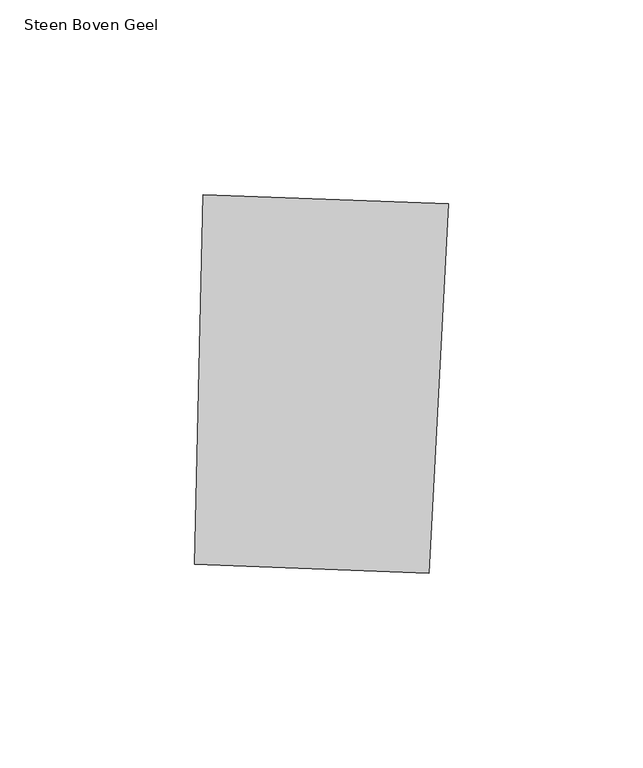
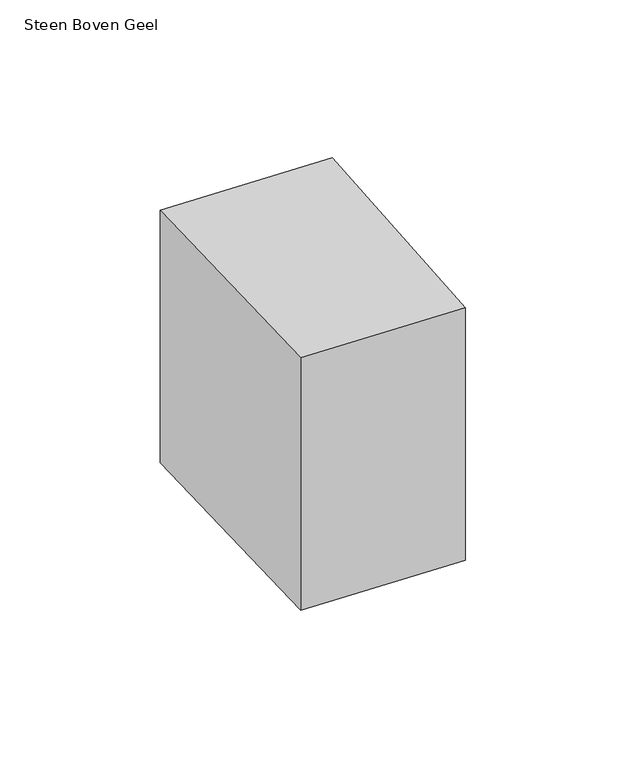
"""IFC4 building model written with IfcOpenShell, lengths in millimetres: proxy geometry, 00_GMA_steen_versie_4 : Steen Boven Geel."""

from ifc_helpers import new_model, si_unit, origin, origin_with_axes, place, context, project, spatial, polyline, outline, extrude, source, transform, mapped, element, save


def steen_boven_geel_c5bd7e60(model_context):
    return source(origin(), model_context, "Body", "SweptSolid", [
        extrude(outline(polyline([(103.188277, 118.7224772), (98.1883411, 23.8434493), (37.9319681, 26.1364041), (40.1569738, 121.1210273), (103.188277, 118.7224772)])), origin_with_axes(), (0.0, 0.0, 1.0), 100.0),
    ])


if __name__ == "__main__":
    model = new_model("IFC4")
    model_context = context("Model", 3, world=origin())
    ifc_project = project(units=[si_unit("LENGTHUNIT", "METRE", prefix="MILLI")], contexts=[model_context])
    site = spatial("IfcSite", under=ifc_project)
    building = spatial("IfcBuilding", under=site)
    placement = place(None, origin())
    steen_boven_geel_shape = steen_boven_geel_c5bd7e60(model_context)
    element("IfcBuildingElementProxy", 1, Name="00_GMA_steen_versie_4 : Steen Boven Geel", ObjectType="00_GMA_steen_versie_4 : Steen Boven Geel", at=placement, inside=building, context=model_context, shape_type="MappedRepresentation", body=[
        mapped(steen_boven_geel_shape, transform((0.0, 0.0, 0.0), x_axis=(1.0, 0.0, 0.0), y_axis=(0.0, 1.0, 0.0), z_axis=(0.0, 0.0, 1.0))),
    ])
    save(model, "model.ifc")

# Revit data of these elements
# Type "00_GMA_steen_versie_4 : Steen Boven Geel"
#   StootVoegHalfBoven [instance default] = 5 mm
#   StootVoegHalf [instance default] = 5 mm
#   StootVoegBreedteOnder = 10 mm
#   StootVoegBreedteBoven = 10 mm
#   Steendikte = 100 mm
#   LintVoegOnderHalf = 5 mm
#   LintVoegOnder = 10 mm
#   LintVoegBovenHalf = 0 mm
#   LintVoegBoven = 0 mm
#   materiaal = 21_steen_geel
#   MateriaalVoeg = none
#   Default Elevation = 0
# Element 1 (IfcBuildingElementProxy, "00_GMA_steen_versie_4 : Steen Boven Geel")
#   Materials on its faces: "21_steen_geel"
# Materials
#   "21_steen_geel": class "Unassigned", colour RGB 202 202 0, transparency 0, Cost = 0
